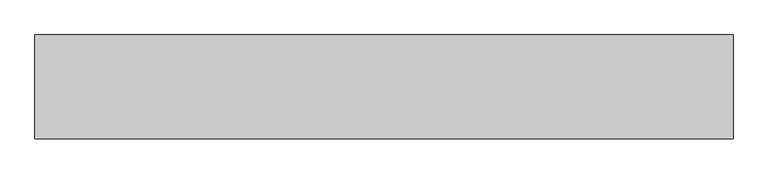
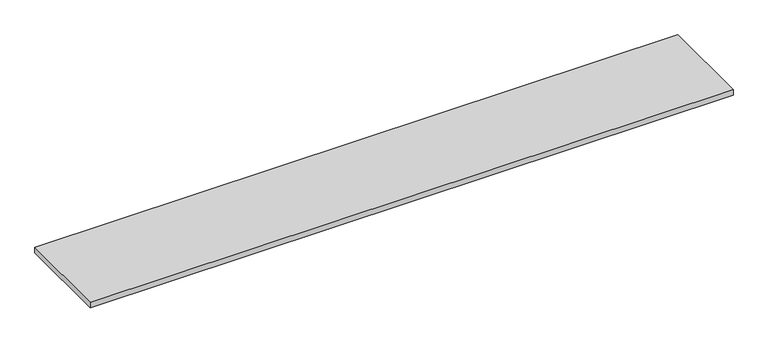
"""IFC4 building model written with IfcOpenShell, lengths in millimetres: furniture geometry, OD_CW_Countertop : OD_CW_Countertop."""

from ifc_helpers import new_model, si_unit, frame, origin, place, context, project, spatial, polyline, outline, extrude, source, transform, mapped, element, save


def furniture_75740181(model_context):
    return source(origin(), model_context, "Body", "SweptSolid", [
        extrude(outline(polyline([(18.7377049, -609.6), (18.7377049, 25.4), (4285.9377049, 25.4), (4285.9377049, -609.6), (18.7377049, -609.6)])), frame((0.0, 0.0, 965.2), z_axis=(0.0, 0.0, 1.0), x_axis=(1.0, 0.0, 0.0)), (0.0, 0.0, 1.0), 38.1),
    ])


if __name__ == "__main__":
    model = new_model("IFC4")
    model_context = context("Model", 3, world=origin())
    ifc_project = project(units=[si_unit("LENGTHUNIT", "METRE", prefix="MILLI")], contexts=[model_context])
    site = spatial("IfcSite", under=ifc_project)
    building = spatial("IfcBuilding", under=site)
    placement = place(None, origin())
    furniture_shape = furniture_75740181(model_context)
    element("IfcFurniture", 1, ObjectType="OD_CW_Countertop : OD_CW_Countertop", at=placement, inside=building, context=model_context, shape_type="MappedRepresentation", body=[
        mapped(furniture_shape, transform((0.0, 0.0, 0.0), x_axis=(1.0, 0.0, 0.0), y_axis=(0.0, 1.0, 0.0), z_axis=(0.0, 0.0, 1.0))),
    ])
    save(model, "model.ifc")

# Revit data of these elements
# Type "OD_CW_Countertop : OD_CW_Countertop"
#   OD_CW_Width [instance default] = 2' - 9"
#   OD_CW_Off Floor [instance default] = 3' - 2"
#   OD_CW_Length [instance default] = 6' - 9"
#   OD_CW_Height [instance default] = 7' - 0"
#   Depth = 2' - 0"
#   Height = 3' - 0"
#   Width = 4' - 0"
#   OD_CW_Material_Countertop [instance default] = none
# Element 1 (IfcFurniture, "OD_CW_Countertop : OD_CW_Countertop")
#   OD_CW_Width = 2' - 1"
#   OD_CW_Length = 14' - 0"
#   OD_CW_Height = 0' - 1 1/2"
#   Materials on its faces: "CASEWORK"
# Materials
#   "CASEWORK": class "Generic", colour RGB 181 181 181, transparency 0, Cost = 0
